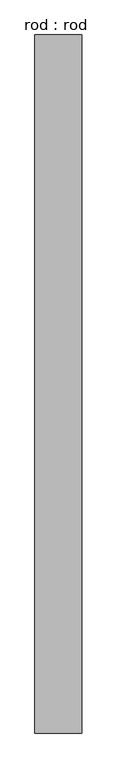
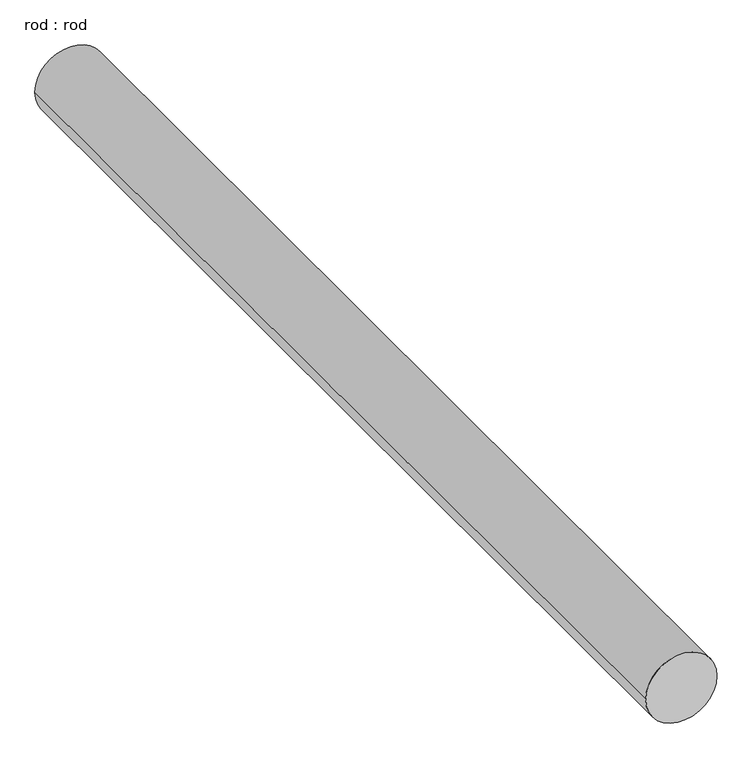
"""IFC4 building model written with IfcOpenShell, lengths in millimetres: proxy geometry, rod : rod."""

from ifc_helpers import new_model, si_unit, point, frame, frame_2d, origin, place, context, project, spatial, circle_curve, trimmed, segment, composite_curve, outline, extrude, source, transform, mapped, element, save


def rod_rod_57927dc1(model_context):
    return source(origin(), model_context, "Body", "SweptSolid", [
        extrude(outline(composite_curve([segment(trimmed(circle_curve(frame_2d((0.0108462, 0.0)), 200.0), [point((0.0108462, 200.0))], [point((0.0108462, -200.0))], False, "CARTESIAN"), True, "CONTINUOUS"), segment(trimmed(circle_curve(frame_2d((0.0108462, 0.0)), 200.0), [point((0.0108462, -200.0))], [point((0.0108462, 200.0))], False, "CARTESIAN"), True, "CONTINUOUS")], self_intersect=False)), frame((0.0, 1119.0909578, 0.0), z_axis=(0.0, 1.0, 0.0), x_axis=(0.0, 0.0, 1.0)), (0.0, 0.0, 1.0), 5947.2753151),
    ])


if __name__ == "__main__":
    model = new_model("IFC4")
    model_context = context("Model", 3, world=origin())
    ifc_project = project(units=[si_unit("LENGTHUNIT", "METRE", prefix="MILLI")], contexts=[model_context])
    site = spatial("IfcSite", under=ifc_project)
    building = spatial("IfcBuilding", under=site)
    placement = place(None, origin())
    rod_rod_shape = rod_rod_57927dc1(model_context)
    element("IfcBuildingElementProxy", 1, Name="rod : rod", ObjectType="rod : rod", at=placement, inside=building, context=model_context, shape_type="MappedRepresentation", body=[
        mapped(rod_rod_shape, transform((0.0, 0.0, 0.0), x_axis=(1.0, 0.0, 0.0), y_axis=(0.0, 1.0, 0.0), z_axis=(0.0, 0.0, 1.0))),
    ])
    save(model, "model.ifc")

# Revit data of these elements
# Type "rod : rod"
#   Default Elevation = 0
